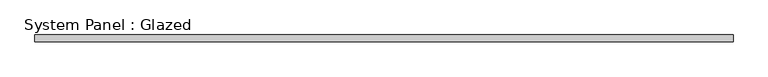
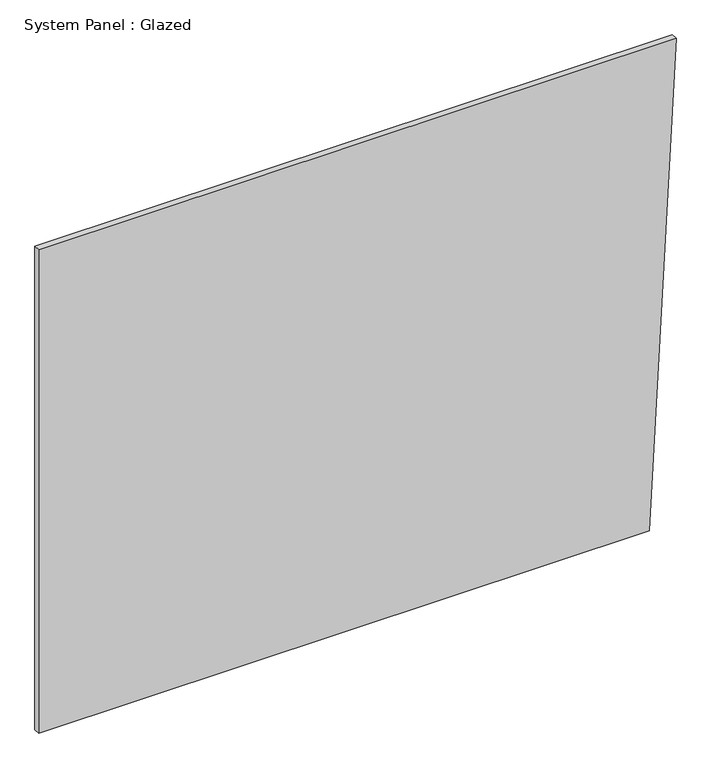
"""IFC4 building model written with IfcOpenShell, lengths in millimetres: plate geometry, System Panel : Glazed."""

from ifc_helpers import new_model, si_unit, frame, origin, place, context, project, spatial, polyline, outline, extrude, source, transform, mapped, element, save


def system_panel_glazed_b312656f(model_context):
    return source(origin(), model_context, "Body", "SweptSolid", [
        extrude(outline(polyline([(0.0, -1300.5178239), (0.0, 1191.3775408), (2085.3785982, 1300.5178239), (2085.3785982, -1300.5178239), (0.0, -1300.5178239)])), frame((0.0, -44.45, 0.0), z_axis=(0.0, 1.0, 0.0), x_axis=(0.0, 0.0, 1.0)), (0.0, 0.0, 1.0), 25.4),
    ])


if __name__ == "__main__":
    model = new_model("IFC4")
    model_context = context("Model", 3, world=origin())
    ifc_project = project(units=[si_unit("LENGTHUNIT", "METRE", prefix="MILLI")], contexts=[model_context])
    site = spatial("IfcSite", under=ifc_project)
    building = spatial("IfcBuilding", under=site)
    placement = place(None, origin())
    system_panel_glazed_shape = system_panel_glazed_b312656f(model_context)
    element("IfcPlate", 1, ObjectType="System Panel : Glazed", at=placement, inside=building, context=model_context, shape_type="MappedRepresentation", body=[
        mapped(system_panel_glazed_shape, transform((0.0, 0.0, 0.0), x_axis=(1.0, 0.0, 0.0), y_axis=(0.0, 1.0, 0.0), z_axis=(0.0, 0.0, 1.0))),
    ])
    save(model, "model.ifc")

# Revit data of these elements
# Type "System Panel : Glazed"
#   Construction Type Id = "GSP4R"
#   Analytic Construction = "1/8 in Pilkington single glazing"
#   Visual Light Transmittance = 0.9
#   Solar Heat Gain Coefficient = 0.86
#   Heat Transfer Coefficient (U) = 1.18115 BTU/(h·ft²·°F)
#   Define Thermal Properties by = 1
# Element 1 (IfcPlate, "System Panel : Glazed")
#   Materials on its faces: "Glass"
# Materials
#   "Glass": class "Glass", colour RGB 0 128 192, transparency 0.75, Description = "Soda Lime Glass", Cost = 0
